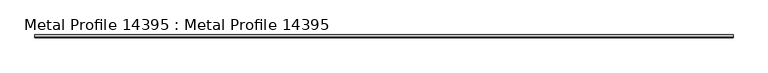
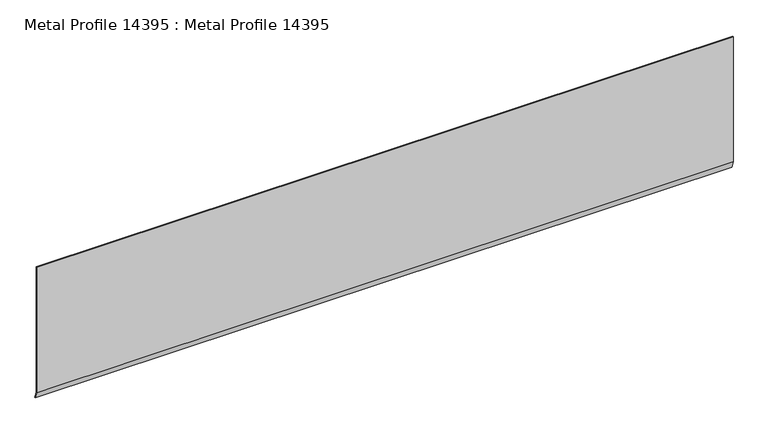
"""IFC4 building model written with IfcOpenShell, lengths in millimetres: proxy geometry, Metal Profile 14395 : Metal Profile 14395."""

from ifc_helpers import new_model, si_unit, frame, origin, place, context, project, spatial, polyline, outline, extrude, source, transform, mapped, element, save


def metal_profile_14395_metal_profile_14395_1ea8b647(model_context):
    return source(origin(), model_context, "Body", "SweptSolid", [
        extrude(outline(polyline([(2292.8641987, 44712.1642551), (2294.8641987, 44712.1642551), (2294.8641987, 44332.1642551), (2301.2291968, 44312.5130547), (2299.3265136, 44311.8967781), (2292.8641987, 44331.8484331), (2292.8641987, 44712.1642551)])), frame((6470.1467506, 0.0, 0.0), z_axis=(1.0, 0.0, 0.0), x_axis=(0.0, 1.0, 0.0)), (0.0, 0.0, 1.0), 1999.85),
    ])


if __name__ == "__main__":
    model = new_model("IFC4")
    model_context = context("Model", 3, world=origin())
    ifc_project = project(units=[si_unit("LENGTHUNIT", "METRE", prefix="MILLI")], contexts=[model_context])
    site = spatial("IfcSite", under=ifc_project)
    building = spatial("IfcBuilding", under=site)
    placement = place(None, origin())
    metal_profile_14395_metal_profile_14395_shape = metal_profile_14395_metal_profile_14395_1ea8b647(model_context)
    element("IfcBuildingElementProxy", 1, Name="Metal Profile 14395 : Metal Profile 14395", ObjectType="Metal Profile 14395 : Metal Profile 14395", at=placement, inside=building, context=model_context, shape_type="MappedRepresentation", body=[
        mapped(metal_profile_14395_metal_profile_14395_shape, transform((0.0, 0.0, 0.0), x_axis=(1.0, 0.0, 0.0), y_axis=(0.0, 1.0, 0.0), z_axis=(0.0, 0.0, 1.0))),
    ])
    save(model, "model.ifc")

# Revit data of these elements
# Type "Metal Profile 14395 : Metal Profile 14395"
#   NameOverride = "Metal Profile"
# Element 1 (IfcBuildingElementProxy, "Metal Profile 14395 : Metal Profile 14395")
#   Materials on its faces: "20 GA. CONTINUOUS CLEAT"
# Materials
#   "20 GA. CONTINUOUS CLEAT": class "Unassigned", colour RGB 245 226 176, transparency 0, Cost = 0
